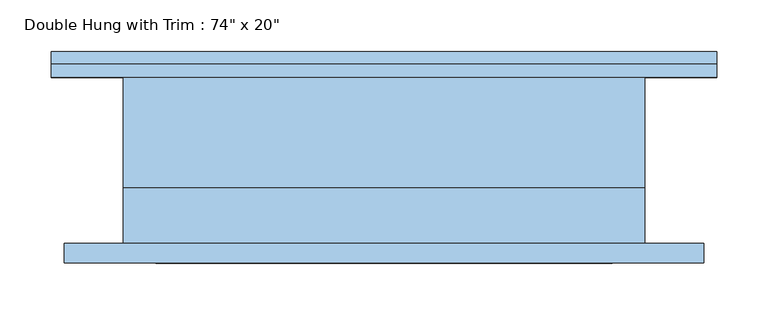
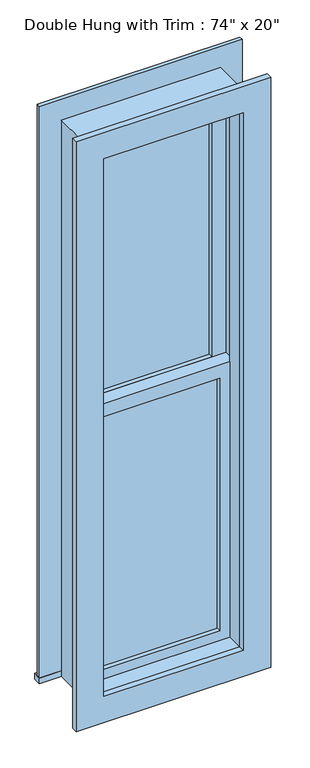
"""IFC4 building model written with IfcOpenShell, lengths in millimetres: window geometry."""

from ifc_helpers import new_model, si_unit, frame, origin, place, context, project, spatial, polyline, outline, extrude, source, transform, mapped, element, save


def window_bad96840(model_context):
    return source(origin(), model_context, "Body", "SweptSolid", [
        extrude(outline(polyline([(-190.5, 1.5875), (190.5, 1.5875), (190.5, -11.1125), (-190.5, -11.1125), (-190.5, 1.5875)])), frame((0.0, 0.0, 571.5), z_axis=(0.0, 0.0, 1.0), x_axis=(1.0, 0.0, 0.0)), (0.0, 0.0, 1.0), 854.075),
        extrude(outline(polyline([(1470.025, -234.95), (527.05, -234.95), (527.05, 234.95), (1470.025, 234.95), (1470.025, -234.95)]), holes=[polyline([(1425.575, -190.5), (1425.575, 190.5), (571.5, 190.5), (571.5, -190.5), (1425.575, -190.5)])]), frame((0.0, -26.9875, 0.0), z_axis=(0.0, 1.0, 0.0), x_axis=(0.0, 0.0, 1.0)), (0.0, 0.0, 1.0), 44.45),
        extrude(outline(polyline([(-323.85, 106.3625), (323.85, 106.3625), (323.85, 80.9625), (-323.85, 80.9625), (-323.85, 106.3625)])), frame((0.0, 0.0, 508.0), z_axis=(0.0, 0.0, 1.0), x_axis=(1.0, 0.0, 0.0)), (0.0, 0.0, 1.0), 19.05),
        extrude(outline(polyline([(2368.55, -234.95), (2368.55, 234.95), (527.05, 234.95), (527.05, 323.85), (2457.45, 323.85), (2457.45, -323.85), (527.05, -323.85), (527.05, -234.95), (2368.55, -234.95)])), frame((0.0, 80.9625, 0.0), z_axis=(0.0, 1.0, 0.0), x_axis=(0.0, 0.0, 1.0)), (0.0, 0.0, 1.0), 12.7),
        extrude(outline(polyline([(2444.75, 311.15), (2444.75, -311.15), (450.85, -311.15), (450.85, 311.15), (2444.75, 311.15)]), holes=[polyline([(2355.85, 222.25), (539.75, 222.25), (539.75, -222.25), (2355.85, -222.25), (2355.85, 222.25)])]), frame((0.0, -100.0125, 0.0), z_axis=(0.0, 1.0, 0.0), x_axis=(0.0, 0.0, 1.0)), (0.0, 0.0, 1.0), 19.05),
        extrude(outline(polyline([(190.5, 33.3375), (-190.5, 33.3375), (-190.5, 46.0375), (190.5, 46.0375), (190.5, 33.3375)])), frame((0.0, 0.0, 1470.025), z_axis=(0.0, 0.0, 1.0), x_axis=(1.0, 0.0, 0.0)), (0.0, 0.0, 1.0), 854.075),
        extrude(outline(polyline([(2368.55, -234.95), (1425.575, -234.95), (1425.575, 234.95), (2368.55, 234.95), (2368.55, -234.95)]), holes=[polyline([(2324.1, -190.5), (2324.1, 190.5), (1470.025, 190.5), (1470.025, -190.5), (2324.1, -190.5)])]), frame((0.0, 17.4625, 0.0), z_axis=(0.0, 1.0, 0.0), x_axis=(0.0, 0.0, 1.0)), (0.0, 0.0, 1.0), 44.45),
        extrude(outline(polyline([(2387.6, -254.0), (508.0, -254.0), (508.0, 254.0), (2387.6, 254.0), (2387.6, -254.0)]), holes=[polyline([(2355.85, -222.25), (2355.85, 222.25), (539.75, 222.25), (539.75, -222.25), (2355.85, -222.25)])]), frame((0.0, -80.9625, 0.0), z_axis=(0.0, 1.0, 0.0), x_axis=(0.0, 0.0, 1.0)), (0.0, 0.0, 1.0), 53.975),
        extrude(outline(polyline([(2387.6, 254.0), (2387.6, -254.0), (508.0, -254.0), (508.0, 254.0), (2387.6, 254.0)]), holes=[polyline([(2368.55, 234.95), (527.05, 234.95), (527.05, -234.95), (2368.55, -234.95), (2368.55, 234.95)])]), frame((0.0, -26.9875, 0.0), z_axis=(0.0, 1.0, 0.0), x_axis=(0.0, 0.0, 1.0)), (0.0, 0.0, 1.0), 107.95),
    ])


if __name__ == "__main__":
    model = new_model("IFC4")
    model_context = context("Model", 3, world=origin())
    ifc_project = project(units=[si_unit("LENGTHUNIT", "METRE", prefix="MILLI")], contexts=[model_context])
    site = spatial("IfcSite", under=ifc_project)
    building = spatial("IfcBuilding", under=site)
    placement = place(None, origin())
    window_shape = window_bad96840(model_context)
    element("IfcWindow", 1, ObjectType="Double Hung with Trim : 74\" x 20\"", at=placement, inside=building, context=model_context, shape_type="MappedRepresentation", body=[
        mapped(window_shape, transform((0.0, 0.0, 0.0), x_axis=(1.0, 0.0, 0.0), y_axis=(0.0, 1.0, 0.0), z_axis=(0.0, 0.0, 1.0))),
    ])
    save(model, "model.ifc")

# Revit data of these elements
# Type "Double Hung with Trim : 74\" x 20\""
#   Type Mark = "56"
#   COBie.Type.CreatedBy = "doug.wood@us.ibm.com"
#   COBie.Type.CreatedOn = "2016-04-14T02:07:26"
#   COBie.Type.Name = "Windows_Double Hung with Trim_74\" x 20\"_56"
#   COBie.Type.Category = "23-30 20 17 17 14 : Double-Hung Windows"
#   COBie.Type.Description = "Double Hung with Trim_74\" x 20\""
#   COBie.Type.Manufacturer = ""
#   COBie.Type.ModelNumber = ""
#   Construction Type Id = "GSP4R"
#   Assembly Code = "B2020100"
#   Analytic Construction = "1/8 in Pilkington single glazing"
#   COBie.Type.ReplacementCost = 0
#   Visual Light Transmittance = 0.9
#   Solar Heat Gain Coefficient = 0.78
#   Heat Transfer Coefficient (U) = 3.6886 W/(m²·K)
#   Height = 6' - 2"
#   Default Sill Height = 1' - 8"
#   Trim Projection - Ext. = 0' - 0 1/2"
#   Trim Projection - Int. = 0' - 0 3/4"
#   Trim Width - Exterior = 0' - 3 1/2"
#   Trim Width - Interior = 0' - 3 1/2"
#   Width = 1' - 8"
#   Window Inset = 0' - 0 3/4"
#   COBie.Type = no
#   Glass Pane Material = Glass
#   Sash Material = Sash - White
#   Trim Exterior Material = Trim - White
#   Trim Interior Material = Trim - White
#   Wall Closure = (empty or 0)
# Element 1 (IfcWindow, "Double Hung with Trim : 74\" x 20\"")
#   Materials on its faces: "Sash - White", "Trim - White", "Glass"
# Materials
#   "Glass": class "Glass", colour RGB 0 128 192, transparency 0.75, Description = "Soda Lime Glass", Cost = 0
#   "Sash - White": class "Wood", colour RGB 255 255 255, transparency 0, Cost = 0
#   "Trim - White": class "Wood", colour RGB 255 255 255, transparency 0, Cost = 0
